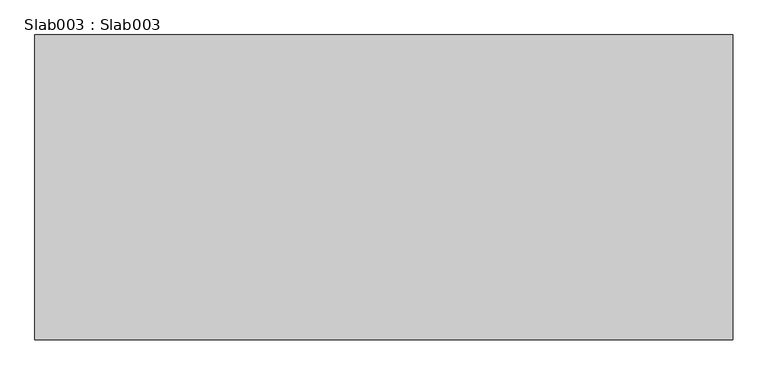
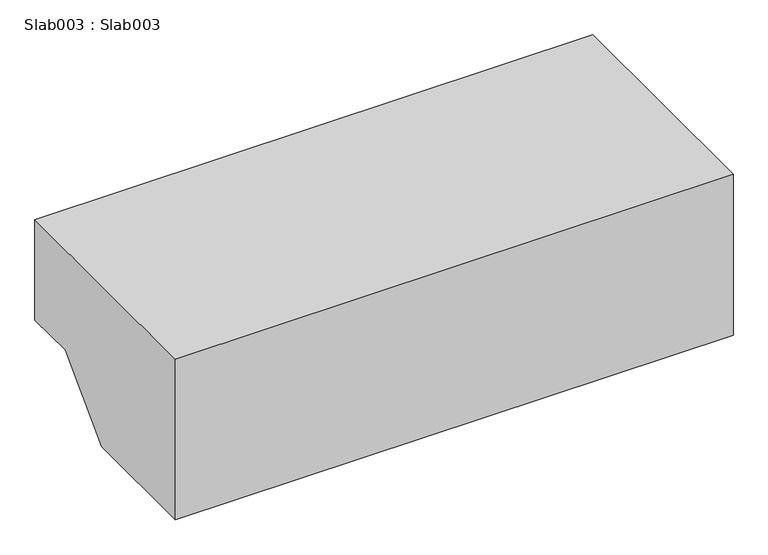
"""IFC4 building model written with IfcOpenShell, lengths in millimetres: proxy geometry, Slab003 : Slab003."""

import ifcopenshell
import ifcopenshell.guid

model = None  # the IFC model being written
_history = None  # IfcOwnerHistory: only IFC2X3 demands one
_inside = {}  # id of a spatial element -> (the spatial element, [elements in it])
_under = {}  # id of a project, library or spatial element -> (it, [spatial elements below it])
_declared = {}  # id of a project -> (the project, [libraries it declares])
_typed = {}  # id of a type object -> (the type object, [elements of that type])
_made_of = {}  # id of a material, layer set ... -> (it, [elements and type objects made of it])


def new_model(schema):
    """Start an empty IFC model of exactly this schema.

    Asked for "IFC4X3", IfcOpenShell would pick the latest addendum, in which some entities
    have other attributes; the version numbers below select the first issue.
    IFC2X3 requires an IfcOwnerHistory on every rooted entity: one is made here for all.
    """
    global model, _history
    if schema == "IFC4X3":
        model = ifcopenshell.file(schema_version=(4, 3, 0, 0))
    else:
        model = ifcopenshell.file(schema=schema)
    _inside.clear()
    _under.clear()
    _declared.clear()
    _typed.clear()
    _made_of.clear()
    _history = None
    if model.schema == "IFC2X3":
        org = make("IfcOrganization", Name="unknown")
        user = make(
            "IfcPersonAndOrganization",
            ThePerson=make("IfcPerson", FamilyName="unknown"),
            TheOrganization=org,
        )
        app = make(
            "IfcApplication",
            ApplicationDeveloper=org,
            Version="unknown",
            ApplicationFullName="unknown",
            ApplicationIdentifier="unknown",
        )
        _history = make(
            "IfcOwnerHistory",
            OwningUser=user,
            OwningApplication=app,
            ChangeAction="ADDED",
            CreationDate=0,
        )
    return model


def make(cls, **values):
    """One entity of the class cls with the attributes given. An attribute that is None is left unset."""
    return model.create_entity(
        cls, **{name: value for name, value in values.items() if value is not None}
    )


def rooted(cls, **values):
    """An entity with a GlobalId (a new one), such as an element, a storey or a relation."""
    return make(cls, GlobalId=ifcopenshell.guid.new(), OwnerHistory=_history, **values)


def si_unit(unit_type, name, prefix=None):
    """IfcSIUnit, for example si_unit("LENGTHUNIT", "METRE", prefix="MILLI")."""
    return make("IfcSIUnit", UnitType=unit_type, Prefix=prefix, Name=name)


def assignment(units):
    """IfcUnitAssignment: the units of a project."""
    return None if units is None else make("IfcUnitAssignment", Units=units)


def point(xyz):
    """IfcCartesianPoint."""
    return None if xyz is None else make("IfcCartesianPoint", Coordinates=xyz)


def direction(xyz):
    """IfcDirection."""
    return None if xyz is None else make("IfcDirection", DirectionRatios=xyz)


def frame(location, z_axis=None, x_axis=None):
    """IfcAxis2Placement3D, a coordinate frame: its origin and axes. An axis left out is left unset."""
    return make(
        "IfcAxis2Placement3D",
        Location=point(location),
        Axis=direction(z_axis),
        RefDirection=direction(x_axis),
    )


def origin():
    """The frame at (0, 0, 0) with its axes left unset."""
    return frame((0.0, 0.0, 0.0))


def place(relative_to, where):
    """IfcLocalPlacement: puts the frame where relative to a parent placement (None: the world)."""
    return make(
        "IfcLocalPlacement", PlacementRelTo=relative_to, RelativePlacement=where
    )


def context(
    kind, dimensions, precision=None, world=None, true_north=None, identifier=None
):
    """IfcGeometricRepresentationContext, for example the 3D "Model" context."""
    return make(
        "IfcGeometricRepresentationContext",
        ContextIdentifier=identifier,
        ContextType=kind,
        CoordinateSpaceDimension=dimensions,
        Precision=precision,
        WorldCoordinateSystem=world,
        TrueNorth=true_north,
    )


def project(units=None, contexts=None):
    """IfcProject with its units and contexts."""
    return rooted(
        "IfcProject",
        Name="project",
        RepresentationContexts=contexts,
        UnitsInContext=assignment(units),
    )


def spatial(cls, under=None, at=None, **own):
    """A site, building, storey or space (cls), placed at a placement, below another one or the project."""
    s = rooted(cls, ObjectPlacement=at, **own)
    if under is not None:
        _under.setdefault(under.id(), (under, []))[1].append(s)
    return s


def polyline(points):
    """IfcPolyline through the points."""
    return make("IfcPolyline", Points=[point(p) for p in points])


def outline(outer, holes=None, kind="AREA"):
    """IfcArbitraryClosedProfileDef: a profile drawn as a closed curve; with holes, ...WithVoids."""
    if holes is None:
        return make("IfcArbitraryClosedProfileDef", ProfileType=kind, OuterCurve=outer)
    return make(
        "IfcArbitraryProfileDefWithVoids",
        ProfileType=kind,
        OuterCurve=outer,
        InnerCurves=holes,
    )


def extrude(swept, where, along, depth):
    """IfcExtrudedAreaSolid: the profile swept, set in the frame where, extruded along a direction by depth."""
    return make(
        "IfcExtrudedAreaSolid",
        SweptArea=swept,
        Position=where,
        ExtrudedDirection=direction(along),
        Depth=depth,
    )


def shape(context_of_items, identifier, shape_type, items):
    """IfcShapeRepresentation: the items that make up one representation, for example the "Body"."""
    return make(
        "IfcShapeRepresentation",
        ContextOfItems=context_of_items,
        RepresentationIdentifier=identifier,
        RepresentationType=shape_type,
        Items=items,
    )


def source(mapping_origin, context_of_items, identifier, shape_type, items):
    """IfcRepresentationMap: a shape defined once, which mapped items show again and again."""
    return make(
        "IfcRepresentationMap",
        MappingOrigin=mapping_origin,
        MappedRepresentation=shape(context_of_items, identifier, shape_type, items),
    )


def transform(
    local_origin,
    x_axis=None,
    y_axis=None,
    z_axis=None,
    scale=None,
    scale2=None,
    scale3=None,
    uniform=True,
):
    """IfcCartesianTransformationOperator3D, or its non-uniform kind. x_axis, y_axis, z_axis: its Axis1, 2, 3."""
    if uniform:
        return make(
            "IfcCartesianTransformationOperator3D",
            Axis1=direction(x_axis),
            Axis2=direction(y_axis),
            LocalOrigin=point(local_origin),
            Scale=scale,
            Axis3=direction(z_axis),
        )
    return make(
        "IfcCartesianTransformationOperator3DnonUniform",
        Axis1=direction(x_axis),
        Axis2=direction(y_axis),
        LocalOrigin=point(local_origin),
        Scale=scale,
        Axis3=direction(z_axis),
        Scale2=scale2,
        Scale3=scale3,
    )


def mapped(mapping_source, mapping_target):
    """IfcMappedItem: shows the shape of a source again, moved by a transform."""
    return make(
        "IfcMappedItem", MappingSource=mapping_source, MappingTarget=mapping_target
    )


def made_of(thing, what):
    """Note that an element or type object is made of a material, layer set ...; save() writes the relation."""
    if what is not None:
        _made_of.setdefault(what.id(), (what, []))[1].append(thing)
    return thing


def element(
    cls,
    number,
    at=None,
    inside=None,
    cuts=None,
    type_object=None,
    material=None,
    context=None,
    identifier="Body",
    shape_type=None,
    held_by="IfcProductDefinitionShape",
    body=None,
    shapes=None,
    **own,
):
    """One element of the class cls, such as IfcWall. Its Tag is "e" and its number.

    at: its placement. inside: the storey or other place that contains it. cuts: it is an
    opening in that element (IfcRelVoidsElement). A single representation is given by context,
    identifier, shape_type and body (its items); several are given by shapes. held_by: the class
    of the entity that holds the representations. save() writes the other relations.
    """
    e = rooted(cls, Tag="e%d" % number, ObjectPlacement=at, **own)
    if body is not None:
        shapes = [shape(context, identifier, shape_type, body)]
    if shapes is not None:
        e.Representation = make(held_by, Representations=shapes)
    if inside is not None:
        _inside.setdefault(inside.id(), (inside, []))[1].append(e)
    if cuts is not None:
        rooted(
            "IfcRelVoidsElement", RelatingBuildingElement=cuts, RelatedOpeningElement=e
        )
    if type_object is not None:
        _typed.setdefault(type_object.id(), (type_object, []))[1].append(e)
    return made_of(e, material)


def aggregate(whole, parts):
    """IfcRelAggregates: a whole, such as a stair, and the parts it consists of."""
    return rooted("IfcRelAggregates", RelatingObject=whole, RelatedObjects=parts)


def save(model, path):
    """Write the relations noted so far, then the file.

    IfcRelAggregates (storeys below a building ...), IfcRelContainedInSpatialStructure (elements
    in a storey), IfcRelDefinesByType, IfcRelAssociatesMaterial and IfcRelDeclares: one each for
    every whole, place, type object, material and project.
    """
    for whole, parts in _under.values():
        aggregate(whole, parts)
    for where, things in _inside.values():
        rooted(
            "IfcRelContainedInSpatialStructure",
            RelatedElements=things,
            RelatingStructure=where,
        )
    for kind, things in _typed.values():
        rooted("IfcRelDefinesByType", RelatedObjects=things, RelatingType=kind)
    for what, things in _made_of.values():
        rooted("IfcRelAssociatesMaterial", RelatedObjects=things, RelatingMaterial=what)
    for by, libraries in _declared.values():
        rooted("IfcRelDeclares", RelatingContext=by, RelatedDefinitions=libraries)
    model.write(path)


def slab003_slab003_fddb5df5(model_context):
    return source(origin(), model_context, "Body", "SweptSolid", [
        extrude(outline(polyline([(-4637.5417972, 36531.296), (-3764.7980951, 36531.296), (-3764.7980951, 36150.296), (-3951.7417972, 36150.296), (-4180.3417972, 35921.696), (-4637.5417972, 35921.696), (-4637.5417972, 36531.296)])), frame((12383.0178845, 0.0, 0.0), z_axis=(1.0, 0.0, 0.0), x_axis=(0.0, 1.0, 0.0)), (0.0, 0.0, 1.0), 2000.0),
    ])


if __name__ == "__main__":
    model = new_model("IFC4")
    model_context = context("Model", 3, world=origin())
    ifc_project = project(units=[si_unit("LENGTHUNIT", "METRE", prefix="MILLI")], contexts=[model_context])
    site = spatial("IfcSite", under=ifc_project)
    building = spatial("IfcBuilding", under=site)
    placement = place(None, origin())
    slab003_slab003_shape = slab003_slab003_fddb5df5(model_context)
    element("IfcBuildingElementProxy", 1, Name="Slab003 : Slab003", ObjectType="Slab003 : Slab003", at=placement, inside=building, context=model_context, shape_type="MappedRepresentation", body=[
        mapped(slab003_slab003_shape, transform((0.0, 0.0, 0.0), x_axis=(1.0, 0.0, 0.0), y_axis=(0.0, 1.0, 0.0), z_axis=(0.0, 0.0, 1.0))),
    ])
    save(model, "model.ifc")

# Revit data of these elements
# Type "Slab003 : Slab003"
#   NameOverride = "Slab003"
# Element 1 (IfcBuildingElementProxy, "Slab003 : Slab003")
#   Materials on its faces: "CONCRETE SLAB W/ GRADE BEAM (SEE STRUCT DWGS)"
# Materials
#   "CONCRETE SLAB W/ GRADE BEAM (SEE STRUCT DWGS)": class "Unassigned", colour RGB 128 128 128, transparency 0, Cost = 0
